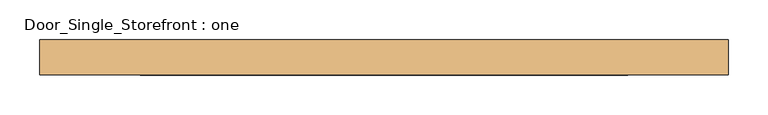
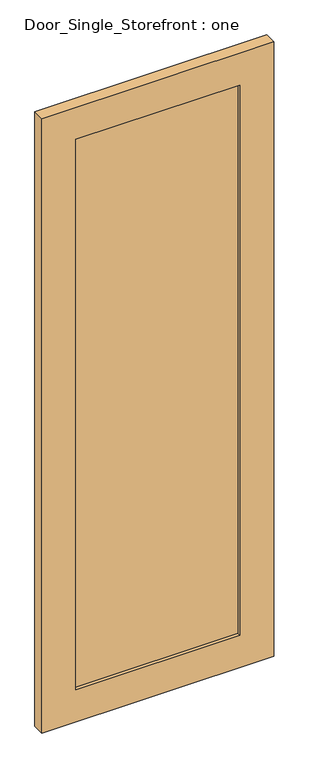
"""IFC4 building model written with IfcOpenShell, lengths in millimetres: door geometry, Door_Single_Storefront : one."""

from ifc_helpers import new_model, si_unit, frame, origin, place, context, project, spatial, polyline, outline, extrude, source, transform, mapped, element, save


def door_single_storefront_one_e0e23135(model_context):
    return source(origin(), model_context, "Body", "SweptSolid", [
        extrude(outline(polyline([(307.18125, -6.35), (-307.18125, -6.35), (-307.18125, 12.7), (307.18125, 12.7), (307.18125, -6.35)])), frame((0.0, 0.0, 127.0), z_axis=(0.0, 0.0, 1.0), x_axis=(1.0, 0.0, 0.0)), (0.0, 0.0, 1.0), 2178.05),
        extrude(outline(polyline([(2432.05, -434.18125), (0.0, -434.18125), (0.0, 434.18125), (2432.05, 434.18125), (2432.05, -434.18125)]), holes=[polyline([(127.0, 307.18125), (127.0, -307.18125), (2305.05, -307.18125), (2305.05, 307.18125), (127.0, 307.18125)])]), frame((0.0, -19.05, 0.0), z_axis=(0.0, 1.0, 0.0), x_axis=(0.0, 0.0, 1.0)), (0.0, 0.0, 1.0), 44.45),
    ])


if __name__ == "__main__":
    model = new_model("IFC4")
    model_context = context("Model", 3, world=origin())
    ifc_project = project(units=[si_unit("LENGTHUNIT", "METRE", prefix="MILLI")], contexts=[model_context])
    site = spatial("IfcSite", under=ifc_project)
    building = spatial("IfcBuilding", under=site)
    placement = place(None, origin())
    door_single_storefront_one_shape = door_single_storefront_one_e0e23135(model_context)
    element("IfcDoor", 1, ObjectType="Door_Single_Storefront : one", at=placement, inside=building, context=model_context, shape_type="MappedRepresentation", body=[
        mapped(door_single_storefront_one_shape, transform((0.0, 0.0, 0.0), x_axis=(1.0, 0.0, 0.0), y_axis=(0.0, 1.0, 0.0), z_axis=(0.0, 0.0, 1.0))),
    ])
    save(model, "model.ifc")

# Revit data of these elements
# Type "Door_Single_Storefront : one"
#   Type Mark = "27"
#   Analytic Construction = "<None>"
#   Stile_Width = 0' - 5"
#   Door_Thickness = 0' - 1 3/4"
#   Door_Offset = 0' - 1"
#   Glass_Material = SAFETY GLAZING
#   Frame_Material = INTERIOR GRADE ALUMINUM STOREFRONT W/ SAFETY GLAZING
#   Function = (empty or 0)
# Element 1 (IfcDoor, "Door_Single_Storefront : one")
#   Materials on its faces: "INTERIOR GRADE ALUMINUM STOREFRONT W/ SAFETY GLAZING", "SAFETY GLAZING"
# Materials
#   "SAFETY GLAZING": class "Glass", colour RGB 142 168 196, transparency 0.75, Description = "Soda Lime Glass", Cost = 0
#   "INTERIOR GRADE ALUMINUM STOREFRONT W/ SAFETY GLAZING": class "Metal", colour RGB 226 226 226, transparency 0, Description = "Aluminum 6061", Cost = 0
